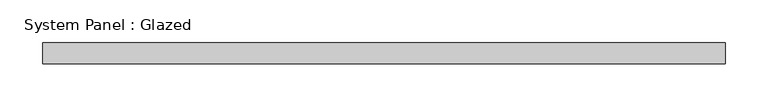
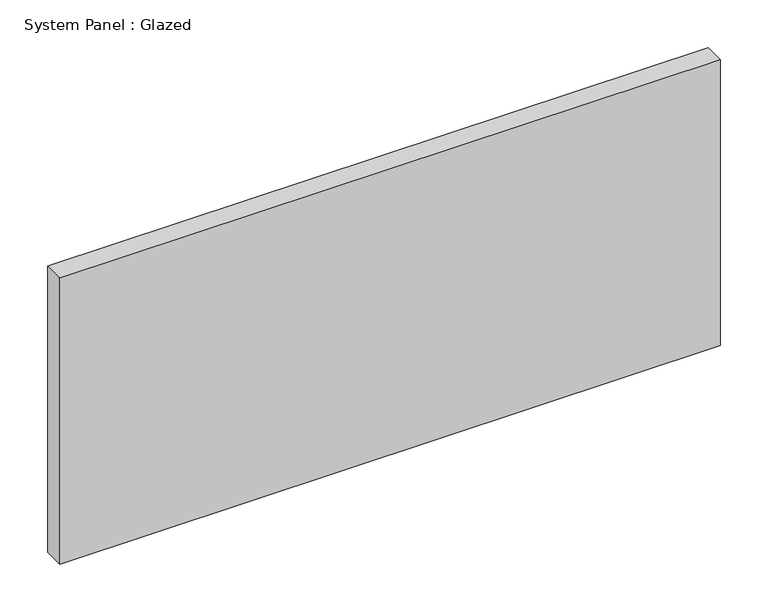
"""IFC4 building model written with IfcOpenShell, lengths in millimetres: plate geometry, System Panel : Glazed."""

from ifc_helpers import new_model, si_unit, origin, origin_with_axes, place, context, project, spatial, polyline, outline, extrude, source, transform, mapped, element, save


def system_panel_glazed_0ea31f09(model_context):
    return source(origin(), model_context, "Body", "SweptSolid", [
        extrude(outline(polyline([(400.0, 24.5), (-400.0, 24.5), (-400.0, 49.5), (400.0, 49.5), (400.0, 24.5)])), origin_with_axes(), (0.0, 0.0, 1.0), 366.6666667),
    ])


if __name__ == "__main__":
    model = new_model("IFC4")
    model_context = context("Model", 3, world=origin())
    ifc_project = project(units=[si_unit("LENGTHUNIT", "METRE", prefix="MILLI")], contexts=[model_context])
    site = spatial("IfcSite", under=ifc_project)
    building = spatial("IfcBuilding", under=site)
    placement = place(None, origin())
    system_panel_glazed_shape = system_panel_glazed_0ea31f09(model_context)
    element("IfcPlate", 1, ObjectType="System Panel : Glazed", at=placement, inside=building, context=model_context, shape_type="MappedRepresentation", body=[
        mapped(system_panel_glazed_shape, transform((0.0, 0.0, 0.0), x_axis=(1.0, 0.0, 0.0), y_axis=(0.0, 1.0, 0.0), z_axis=(0.0, 0.0, 1.0))),
    ])
    save(model, "model.ifc")

# Revit data of these elements
# Element 1 (IfcPlate, "System Panel : Glazed")
#   Materials on its faces: "Glass"
# Materials
#   "Glass": class "Glass", colour RGB 218 227 224, transparency 0.85, Description = "Soda Lime Glass", Cost = 0
